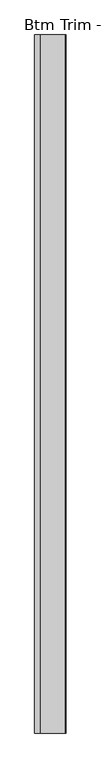
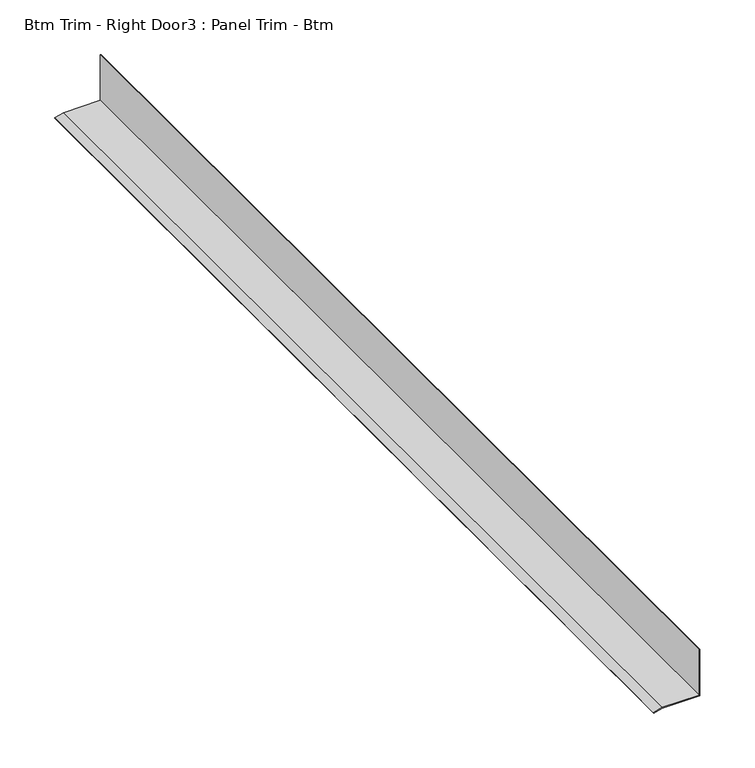
"""IFC4 building model written with IfcOpenShell, lengths in millimetres: proxy geometry, Btm Trim - Right Door3 : Panel Trim - Btm."""

from ifc_helpers import new_model, si_unit, frame, origin, place, context, project, spatial, polyline, outline, extrude, source, transform, mapped, element, save


def btm_trim_right_door3_panel_trim_btm_a276b19c(model_context):
    return source(origin(), model_context, "Body", "SweptSolid", [
        extrude(outline(polyline([(50.8, 587326.1141748), (48.3077022, 587316.8127928), (47.5409986, 587317.0182304), (50.00625, 587326.2186739), (50.00625, 587365.8934739), (101.6, 587365.8934739), (101.6, 587365.1060739), (50.8, 587365.1060739), (50.8, 587326.1141748)])), frame((0.0, -536301.7038841, 0.0), z_axis=(0.0, 1.0, 0.0), x_axis=(0.0, 0.0, 1.0)), (0.0, 0.0, 1.0), 1094.5749),
    ])


if __name__ == "__main__":
    model = new_model("IFC4")
    model_context = context("Model", 3, world=origin())
    ifc_project = project(units=[si_unit("LENGTHUNIT", "METRE", prefix="MILLI")], contexts=[model_context])
    site = spatial("IfcSite", under=ifc_project)
    building = spatial("IfcBuilding", under=site)
    placement = place(None, origin())
    btm_trim_right_door3_panel_trim_btm_shape = btm_trim_right_door3_panel_trim_btm_a276b19c(model_context)
    element("IfcBuildingElementProxy", 1, Name="Btm Trim - Right Door3 : Panel Trim - Btm", ObjectType="Btm Trim - Right Door3 : Panel Trim - Btm", at=placement, inside=building, context=model_context, shape_type="MappedRepresentation", body=[
        mapped(btm_trim_right_door3_panel_trim_btm_shape, transform((0.0, 0.0, 0.0), x_axis=(1.0, 0.0, 0.0), y_axis=(0.0, 1.0, 0.0), z_axis=(0.0, 0.0, 1.0))),
    ])
    save(model, "model.ifc")

# Revit data of these elements
# Element 1 (IfcBuildingElementProxy, "Btm Trim - Right Door3 : Panel Trim - Btm")
#   Materials on its faces: "BASE TRIM BY MTL PANEL MFR."
# Materials
#   "BASE TRIM BY MTL PANEL MFR.": class "Generic", colour RGB 239 242 240, transparency 0, Cost = 0
